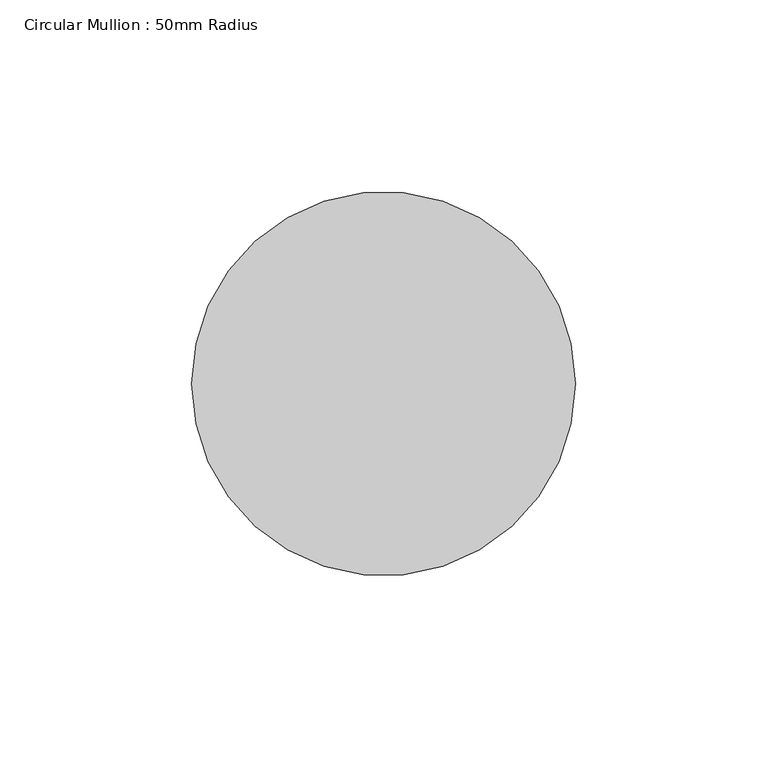
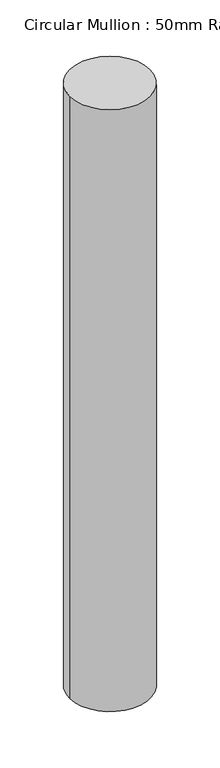
"""IFC4 building model written with IfcOpenShell, lengths in millimetres: member geometry, Circular Mullion : 50mm Radius."""

from ifc_helpers import new_model, si_unit, point, frame, origin, origin_2d, place, context, project, spatial, circle_curve, trimmed, segment, composite_curve, outline, extrude, source, transform, mapped, element, save


def circular_mullion_50mm_radius_0d5fe0ad(model_context):
    return source(origin(), model_context, "Body", "SweptSolid", [
        extrude(outline(composite_curve([segment(trimmed(circle_curve(origin_2d(), 50.0), [point((50.0, 0.0))], [point((-50.0, 0.0))], False, "CARTESIAN"), True, "CONTINUOUS"), segment(trimmed(circle_curve(origin_2d(), 50.0), [point((-50.0, 0.0))], [point((50.0, 0.0))], False, "CARTESIAN"), True, "CONTINUOUS")], self_intersect=False)), frame((0.0, 0.0, -789.2464334), z_axis=(0.0, 0.0, 1.0), x_axis=(1.0, 0.0, 0.0)), (0.0, 0.0, 1.0), 789.2464334),
    ])


if __name__ == "__main__":
    model = new_model("IFC4")
    model_context = context("Model", 3, world=origin())
    ifc_project = project(units=[si_unit("LENGTHUNIT", "METRE", prefix="MILLI")], contexts=[model_context])
    site = spatial("IfcSite", under=ifc_project)
    building = spatial("IfcBuilding", under=site)
    placement = place(None, origin())
    circular_mullion_50mm_radius_shape = circular_mullion_50mm_radius_0d5fe0ad(model_context)
    element("IfcMember", 1, ObjectType="Circular Mullion : 50mm Radius", at=placement, inside=building, context=model_context, shape_type="MappedRepresentation", body=[
        mapped(circular_mullion_50mm_radius_shape, transform((0.0, 0.0, 0.0), x_axis=(1.0, 0.0, 0.0), y_axis=(0.0, 1.0, 0.0), z_axis=(0.0, 0.0, 1.0))),
    ])
    save(model, "model.ifc")

# Revit data of these elements
# Type "Circular Mullion : 50mm Radius"
#   built-in parameter 1007350 = 0.164042 (stored number, unit not read)
# Element 1 (IfcMember, "Circular Mullion : 50mm Radius")
#   Materials on its faces: "Aluminium"
# Materials
#   "Aluminium": class "Metal", colour RGB 247 247 247, transparency 0, Description = "Aluminium 6061", Cost = 0
